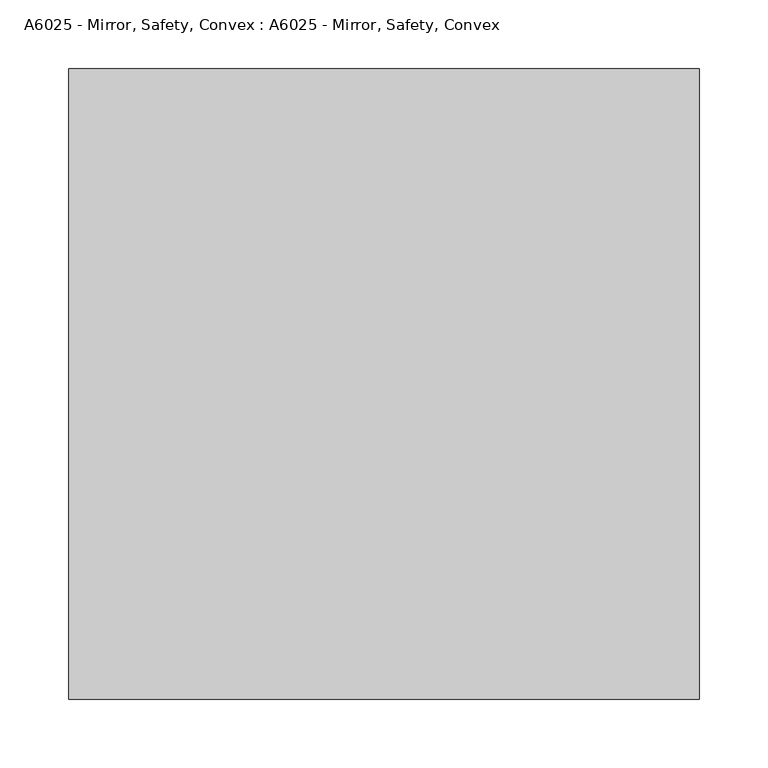
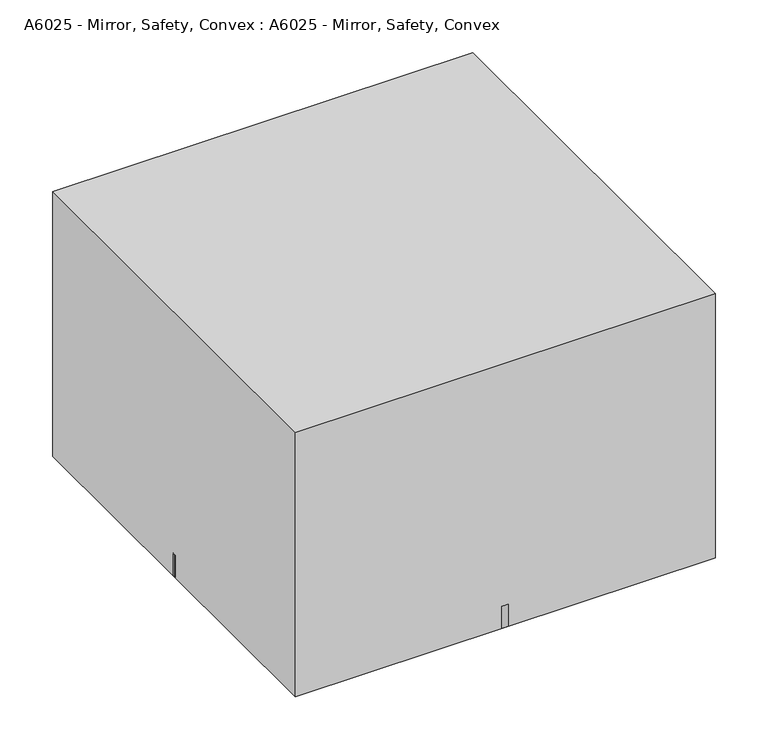
"""IFC4 building model written with IfcOpenShell, lengths in millimetres: proxy geometry, A6025 - Mirror, Safety, Convex : A6025 - Mirror, Safety, Convex."""

import ifcopenshell
import ifcopenshell.guid

model = None  # the IFC model being written
_history = None  # IfcOwnerHistory: only IFC2X3 demands one
_inside = {}  # id of a spatial element -> (the spatial element, [elements in it])
_under = {}  # id of a project, library or spatial element -> (it, [spatial elements below it])
_declared = {}  # id of a project -> (the project, [libraries it declares])
_typed = {}  # id of a type object -> (the type object, [elements of that type])
_made_of = {}  # id of a material, layer set ... -> (it, [elements and type objects made of it])


def new_model(schema):
    """Start an empty IFC model of exactly this schema.

    Asked for "IFC4X3", IfcOpenShell would pick the latest addendum, in which some entities
    have other attributes; the version numbers below select the first issue.
    IFC2X3 requires an IfcOwnerHistory on every rooted entity: one is made here for all.
    """
    global model, _history
    if schema == "IFC4X3":
        model = ifcopenshell.file(schema_version=(4, 3, 0, 0))
    else:
        model = ifcopenshell.file(schema=schema)
    _inside.clear()
    _under.clear()
    _declared.clear()
    _typed.clear()
    _made_of.clear()
    _history = None
    if model.schema == "IFC2X3":
        org = make("IfcOrganization", Name="unknown")
        user = make(
            "IfcPersonAndOrganization",
            ThePerson=make("IfcPerson", FamilyName="unknown"),
            TheOrganization=org,
        )
        app = make(
            "IfcApplication",
            ApplicationDeveloper=org,
            Version="unknown",
            ApplicationFullName="unknown",
            ApplicationIdentifier="unknown",
        )
        _history = make(
            "IfcOwnerHistory",
            OwningUser=user,
            OwningApplication=app,
            ChangeAction="ADDED",
            CreationDate=0,
        )
    return model


def make(cls, **values):
    """One entity of the class cls with the attributes given. An attribute that is None is left unset."""
    return model.create_entity(
        cls, **{name: value for name, value in values.items() if value is not None}
    )


def rooted(cls, **values):
    """An entity with a GlobalId (a new one), such as an element, a storey or a relation."""
    return make(cls, GlobalId=ifcopenshell.guid.new(), OwnerHistory=_history, **values)


def si_unit(unit_type, name, prefix=None):
    """IfcSIUnit, for example si_unit("LENGTHUNIT", "METRE", prefix="MILLI")."""
    return make("IfcSIUnit", UnitType=unit_type, Prefix=prefix, Name=name)


def assignment(units):
    """IfcUnitAssignment: the units of a project."""
    return None if units is None else make("IfcUnitAssignment", Units=units)


def point(xyz):
    """IfcCartesianPoint."""
    return None if xyz is None else make("IfcCartesianPoint", Coordinates=xyz)


def direction(xyz):
    """IfcDirection."""
    return None if xyz is None else make("IfcDirection", DirectionRatios=xyz)


def frame(location, z_axis=None, x_axis=None):
    """IfcAxis2Placement3D, a coordinate frame: its origin and axes. An axis left out is left unset."""
    return make(
        "IfcAxis2Placement3D",
        Location=point(location),
        Axis=direction(z_axis),
        RefDirection=direction(x_axis),
    )


def frame_2d(location, x_axis=None):
    """IfcAxis2Placement2D, a coordinate frame in the plane: its origin and x axis."""
    return make(
        "IfcAxis2Placement2D", Location=point(location), RefDirection=direction(x_axis)
    )


def origin():
    """The frame at (0, 0, 0) with its axes left unset."""
    return frame((0.0, 0.0, 0.0))


def origin_with_axes():
    """The frame at (0, 0, 0) with the z axis (0, 0, 1) and the x axis (1, 0, 0) written out."""
    return frame((0.0, 0.0, 0.0), z_axis=(0.0, 0.0, 1.0), x_axis=(1.0, 0.0, 0.0))


def place(relative_to, where):
    """IfcLocalPlacement: puts the frame where relative to a parent placement (None: the world)."""
    return make(
        "IfcLocalPlacement", PlacementRelTo=relative_to, RelativePlacement=where
    )


def context(
    kind, dimensions, precision=None, world=None, true_north=None, identifier=None
):
    """IfcGeometricRepresentationContext, for example the 3D "Model" context."""
    return make(
        "IfcGeometricRepresentationContext",
        ContextIdentifier=identifier,
        ContextType=kind,
        CoordinateSpaceDimension=dimensions,
        Precision=precision,
        WorldCoordinateSystem=world,
        TrueNorth=true_north,
    )


def project(units=None, contexts=None):
    """IfcProject with its units and contexts."""
    return rooted(
        "IfcProject",
        Name="project",
        RepresentationContexts=contexts,
        UnitsInContext=assignment(units),
    )


def spatial(cls, under=None, at=None, **own):
    """A site, building, storey or space (cls), placed at a placement, below another one or the project."""
    s = rooted(cls, ObjectPlacement=at, **own)
    if under is not None:
        _under.setdefault(under.id(), (under, []))[1].append(s)
    return s


def polyline(points):
    """IfcPolyline through the points."""
    return make("IfcPolyline", Points=[point(p) for p in points])


def circle_curve(where, radius):
    """IfcCircle in the frame where."""
    return make("IfcCircle", Position=where, Radius=radius)


def ellipse_curve(where, semi_axis1, semi_axis2):
    """IfcEllipse in the frame where."""
    return make(
        "IfcEllipse", Position=where, SemiAxis1=semi_axis1, SemiAxis2=semi_axis2
    )


def trimmed(basis, trim1, trim2, sense, master):
    """IfcTrimmedCurve: the piece of a basis curve between two trims."""
    return make(
        "IfcTrimmedCurve",
        BasisCurve=basis,
        Trim1=trim1,
        Trim2=trim2,
        SenseAgreement=sense,
        MasterRepresentation=master,
    )


def segment(curve, same_sense, transition):
    """IfcCompositeCurveSegment."""
    return make(
        "IfcCompositeCurveSegment",
        Transition=transition,
        SameSense=same_sense,
        ParentCurve=curve,
    )


def composite_curve(segments, self_intersect=None):
    """IfcCompositeCurve: segments joined end to end."""
    return make("IfcCompositeCurve", Segments=segments, SelfIntersect=self_intersect)


def outline(outer, holes=None, kind="AREA"):
    """IfcArbitraryClosedProfileDef: a profile drawn as a closed curve; with holes, ...WithVoids."""
    if holes is None:
        return make("IfcArbitraryClosedProfileDef", ProfileType=kind, OuterCurve=outer)
    return make(
        "IfcArbitraryProfileDefWithVoids",
        ProfileType=kind,
        OuterCurve=outer,
        InnerCurves=holes,
    )


def extrude(swept, where, along, depth):
    """IfcExtrudedAreaSolid: the profile swept, set in the frame where, extruded along a direction by depth."""
    return make(
        "IfcExtrudedAreaSolid",
        SweptArea=swept,
        Position=where,
        ExtrudedDirection=direction(along),
        Depth=depth,
    )


def shape(context_of_items, identifier, shape_type, items):
    """IfcShapeRepresentation: the items that make up one representation, for example the "Body"."""
    return make(
        "IfcShapeRepresentation",
        ContextOfItems=context_of_items,
        RepresentationIdentifier=identifier,
        RepresentationType=shape_type,
        Items=items,
    )


def source(mapping_origin, context_of_items, identifier, shape_type, items):
    """IfcRepresentationMap: a shape defined once, which mapped items show again and again."""
    return make(
        "IfcRepresentationMap",
        MappingOrigin=mapping_origin,
        MappedRepresentation=shape(context_of_items, identifier, shape_type, items),
    )


def transform(
    local_origin,
    x_axis=None,
    y_axis=None,
    z_axis=None,
    scale=None,
    scale2=None,
    scale3=None,
    uniform=True,
):
    """IfcCartesianTransformationOperator3D, or its non-uniform kind. x_axis, y_axis, z_axis: its Axis1, 2, 3."""
    if uniform:
        return make(
            "IfcCartesianTransformationOperator3D",
            Axis1=direction(x_axis),
            Axis2=direction(y_axis),
            LocalOrigin=point(local_origin),
            Scale=scale,
            Axis3=direction(z_axis),
        )
    return make(
        "IfcCartesianTransformationOperator3DnonUniform",
        Axis1=direction(x_axis),
        Axis2=direction(y_axis),
        LocalOrigin=point(local_origin),
        Scale=scale,
        Axis3=direction(z_axis),
        Scale2=scale2,
        Scale3=scale3,
    )


def mapped(mapping_source, mapping_target):
    """IfcMappedItem: shows the shape of a source again, moved by a transform."""
    return make(
        "IfcMappedItem", MappingSource=mapping_source, MappingTarget=mapping_target
    )


def made_of(thing, what):
    """Note that an element or type object is made of a material, layer set ...; save() writes the relation."""
    if what is not None:
        _made_of.setdefault(what.id(), (what, []))[1].append(thing)
    return thing


def element(
    cls,
    number,
    at=None,
    inside=None,
    cuts=None,
    type_object=None,
    material=None,
    context=None,
    identifier="Body",
    shape_type=None,
    held_by="IfcProductDefinitionShape",
    body=None,
    shapes=None,
    **own,
):
    """One element of the class cls, such as IfcWall. Its Tag is "e" and its number.

    at: its placement. inside: the storey or other place that contains it. cuts: it is an
    opening in that element (IfcRelVoidsElement). A single representation is given by context,
    identifier, shape_type and body (its items); several are given by shapes. held_by: the class
    of the entity that holds the representations. save() writes the other relations.
    """
    e = rooted(cls, Tag="e%d" % number, ObjectPlacement=at, **own)
    if body is not None:
        shapes = [shape(context, identifier, shape_type, body)]
    if shapes is not None:
        e.Representation = make(held_by, Representations=shapes)
    if inside is not None:
        _inside.setdefault(inside.id(), (inside, []))[1].append(e)
    if cuts is not None:
        rooted(
            "IfcRelVoidsElement", RelatingBuildingElement=cuts, RelatedOpeningElement=e
        )
    if type_object is not None:
        _typed.setdefault(type_object.id(), (type_object, []))[1].append(e)
    return made_of(e, material)


def aggregate(whole, parts):
    """IfcRelAggregates: a whole, such as a stair, and the parts it consists of."""
    return rooted("IfcRelAggregates", RelatingObject=whole, RelatedObjects=parts)


def save(model, path):
    """Write the relations noted so far, then the file.

    IfcRelAggregates (storeys below a building ...), IfcRelContainedInSpatialStructure (elements
    in a storey), IfcRelDefinesByType, IfcRelAssociatesMaterial and IfcRelDeclares: one each for
    every whole, place, type object, material and project.
    """
    for whole, parts in _under.values():
        aggregate(whole, parts)
    for where, things in _inside.values():
        rooted(
            "IfcRelContainedInSpatialStructure",
            RelatedElements=things,
            RelatingStructure=where,
        )
    for kind, things in _typed.values():
        rooted("IfcRelDefinesByType", RelatedObjects=things, RelatingType=kind)
    for what, things in _made_of.values():
        rooted("IfcRelAssociatesMaterial", RelatedObjects=things, RelatingMaterial=what)
    for by, libraries in _declared.values():
        rooted("IfcRelDeclares", RelatingContext=by, RelatedDefinitions=libraries)
    model.write(path)


def plane_surface(at):
    """IfcPlane: the flat surface through the origin of the frame at, square to its z axis."""
    return make("IfcPlane", Position=at)


def revolved_surface(curve, axis_point, axis_direction):
    """IfcSurfaceOfRevolution: the curve turned about the line through axis_point along axis_direction."""
    return make(
        "IfcSurfaceOfRevolution",
        SweptCurve=make("IfcArbitraryOpenProfileDef", ProfileType="CURVE", Curve=curve),
        AxisPosition=make("IfcAxis1Placement", Location=point(axis_point), Axis=direction(axis_direction)),
    )


def advanced_brep(points, edges, surfaces, faces):
    """IfcAdvancedBrep: a solid bounded by faces that lie on surfaces and meet in shared edges.

    An edge is (start, end): straight between two places in points (the first is 0);
    or (start, end, curve); or (start, end, curve, False) where it runs against its curve.
    A face is (place in surfaces, loops), or (place, loops, False) where it looks against
    its surface's normal. A loop lists edges by number (the first is 1), with a minus sign
    where the edge is run from its end to its start. The first loop is the outer one.
    """
    corners = [point(p) for p in points]
    vertices = [make("IfcVertexPoint", VertexGeometry=c) for c in corners]
    made = []
    for start, end, *more in edges:
        made.append(
            make(
                "IfcEdgeCurve",
                EdgeStart=vertices[start],
                EdgeEnd=vertices[end],
                EdgeGeometry=more[0] if more else make("IfcPolyline", Points=[corners[start], corners[end]]),
                SameSense=more[1] if len(more) > 1 else True,
            )
        )
    hull = []
    for where, loops, *sense in faces:
        bounds = []
        for j, loop in enumerate(loops):
            ring = [make("IfcOrientedEdge", EdgeElement=made[abs(k) - 1], Orientation=k > 0) for k in loop]
            bounds.append(
                make(
                    "IfcFaceOuterBound" if j == 0 else "IfcFaceBound",
                    Bound=make("IfcEdgeLoop", EdgeList=ring),
                    Orientation=True,
                )
            )
        hull.append(make("IfcAdvancedFace", Bounds=bounds, FaceSurface=surfaces[where], SameSense=sense[0] if sense else True))
    return make("IfcAdvancedBrep", Outer=make("IfcClosedShell", CfsFaces=hull))


def a6025_mirror_safety_convex_a6025_mirror_safety_convex_4908c988(model_context):
    return source(origin(), model_context, "Body", "SolidModel", [
        advanced_brep(
        [(0.0, -228.6, 25.4), (0.0, -444.5, 25.4), (0.0, -12.7, 25.4), (0.0, -228.6, 127.0)],
        [
            (0, 1),
            (1, 2, circle_curve(frame((0.0, -228.6, 25.4), z_axis=(0.0, 0.0, -1.0), x_axis=(0.0, 1.0, 0.0)), 215.9)),
            (2, 0),
            (2, 1, circle_curve(frame((0.0, -228.6, 25.4), z_axis=(0.0, 0.0, -1.0), x_axis=(0.0, 1.0, 0.0)), 215.9)),
            (1, 3, circle_curve(frame((0.0, -240.4330428, -128.0485341), z_axis=(-1.0, 0.0, 0.0), x_axis=(0.0, 1.0, 0.0)), 255.3228851)),
            (3, 2, circle_curve(frame((0.0, -216.7669572, -128.0485341), z_axis=(-1.0, 0.0, 0.0), x_axis=(0.0, -1.0, 0.0)), 255.3228851)),
        ],
        [
            plane_surface(frame((0.0, -228.6, 25.4), z_axis=(0.0, 0.0, -1.0), x_axis=(0.0, 1.0, 0.0))),
            revolved_surface(trimmed(ellipse_curve(frame((0.0, -216.7669572, -128.0485341), z_axis=(-1.0, 0.0, 0.0), x_axis=(0.0, -1.0, 0.0)), 255.3228851, 255.3228851), [point((0.0, -228.6, 127.0))], [point((0.0, -12.7, 25.4))], True, "CARTESIAN"), (0.0, -228.6, 190.5), (0.0, 0.0, -1.0)),
        ],
        [
            (0, [[1, 2, 3]]),
            (0, [[-3, 4, -1]]),
            (1, [[5, 6, -2]]),
            (1, [[-6, -5, -4]]),
        ],
    ),
        extrude(outline(composite_curve([segment(trimmed(circle_curve(frame_2d((0.0, -228.6)), 228.6), [point((-228.6, -228.6))], [point((228.6, -228.6))], False, "CARTESIAN"), True, "CONTINUOUS"), segment(trimmed(circle_curve(frame_2d((0.0, -228.6)), 228.6), [point((228.6, -228.6))], [point((-228.6, -228.6))], False, "CARTESIAN"), True, "CONTINUOUS")], self_intersect=False)), origin_with_axes(), (0.0, 0.0, 1.0), 25.4),
        extrude(outline(polyline([(228.6, -457.2), (-228.6, -457.2), (-228.6, 0.0), (228.6, 0.0), (228.6, -457.2)])), origin_with_axes(), (0.0, 0.0, 1.0), 304.8),
    ])


if __name__ == "__main__":
    model = new_model("IFC4")
    model_context = context("Model", 3, world=origin())
    ifc_project = project(units=[si_unit("LENGTHUNIT", "METRE", prefix="MILLI")], contexts=[model_context])
    site = spatial("IfcSite", under=ifc_project)
    building = spatial("IfcBuilding", under=site)
    placement = place(None, origin())
    a6025_mirror_safety_convex_a6025_mirror_safety_convex_shape = a6025_mirror_safety_convex_a6025_mirror_safety_convex_4908c988(model_context)
    element("IfcBuildingElementProxy", 1, Name="A6025 - Mirror, Safety, Convex : A6025 - Mirror, Safety, Convex", ObjectType="A6025 - Mirror, Safety, Convex : A6025 - Mirror, Safety, Convex", at=placement, inside=building, context=model_context, shape_type="MappedRepresentation", body=[
        mapped(a6025_mirror_safety_convex_a6025_mirror_safety_convex_shape, transform((0.0, 0.0, 0.0), x_axis=(1.0, 0.0, 0.0), y_axis=(0.0, 1.0, 0.0), z_axis=(0.0, 0.0, 1.0))),
    ])
    save(model, "model.ifc")

# Revit data of these elements
# Project information
#   Room Abbreviation = "BRNP5/BRNP6"
#   Room Description 3-1 = "Seclusion Room (BRNP5)"
#   Room Description 3-2 = "Anteroom, Seclusion (BRNP6)"
#   Room Description 3-3 = "Toilet, Seclusion (TLTP2)"
#   Sheets - Total = "7"
#   Project Issue Date = "Issue Date"
#   Project Status = "Project Status"
#   Client Name = "Owner"
#   Project Address = "Enter address here"
#   Project Name = "Project Name"
#   Project Number = "Project Number"
#   Publication Date = "1-Feb-16"
# Type "A6025 - Mirror, Safety, Convex : A6025 - Mirror, Safety, Convex"
#   Watts2 = "0"
#   Watts1 = "0"
#   Unit_Issue = "EA"
#   UTIL_6_Misc = "-"
#   UTIL_5_NonMedGas = "-"
#   UTIL_4_MiscGas = "-"
#   UTIL_3_MedGas = "-"
#   UTIL_2_Elec = "-"
#   UTIL_1_WaterDrain = "-"
#   Nomenclature = "Mirror, Safety, Convex"
#   NSN = "7105"
#   Location [instance default] = ""
#   JSN = "A6025"
#   Fund_Source_VA = "-"
#   Fund_Source_Navy = "-"
#   Fund_Source_Army = "-"
#   Fund_Source_AF = "-"
#   ELEC_Volts2 = "0"
#   ELEC_Volts1 = "0"
#   ELEC_Phase2 = "0"
#   ELEC_Phase1 = "0"
#   ELEC_HertzSwitch = "0"
#   ELEC_HertzDependent = "0"
#   ELEC_Hertz = "0"
#   ELEC_Amps2 = "0"
#   ELEC_Amps1 = "0"
#   DetailDescription = "Shall be an 18 inch convex circular mirror. It shall provide a 160-degree wide-field viewing area. The mirror shall be made of shatterproof acrylic or unbreakable polycarbonate. Shall come with mounting bracket."
#   CAT_VA = "C"
#   CAT_Navy = "C"
#   CAT_IHS = "-"
#   CAT_Army = "C"
#   CAT_AF = "C"
#   BTUperhour = "0"
#   radius = 0' - 9"
#   Weight_IP = 12
#   Default Elevation = 6' - 6"
#   DIM_Width_IP = 1' - 6"
#   DIM_Height_IP = 1' - 6"
#   DIM_Depth_IP = 1' - 0"
#   Assembly Code = ""
# Element 1 (IfcBuildingElementProxy, "A6025 - Mirror, Safety, Convex : A6025 - Mirror, Safety, Convex")
#   Materials on its faces: "EquipSpace", "Mirror"
# Materials
#   "EquipSpace": class "Unassigned", colour RGB 221 217 195, transparency 0.5
#   "Mirror": class "Unassigned", colour RGB 192 192 192, transparency 0
